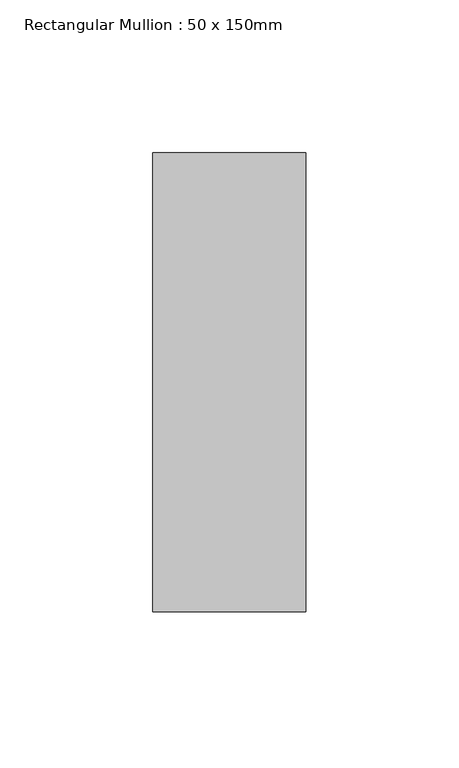
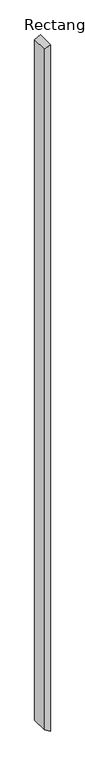
"""IFC4 building model written with IfcOpenShell, lengths in millimetres: member geometry, Rectangular Mullion : 50 x 150mm."""

from ifc_helpers import new_model, si_unit, frame, origin, place, context, project, spatial, polyline, outline, extrude, source, transform, mapped, element, save


def rectangular_mullion_50_x_150mm_85ac93d7(model_context):
    return source(origin(), model_context, "Body", "SweptSolid", [
        extrude(outline(polyline([(0.0, 0.0), (-25.8377402, -50.0), (-6312.9528574, -50.0), (-6342.8393821, 0.0), (0.0, 0.0)])), frame((0.0, -75.0, 0.0), z_axis=(0.0, 1.0, 0.0), x_axis=(0.0, 0.0, 1.0)), (0.0, 0.0, 1.0), 150.0),
    ])


if __name__ == "__main__":
    model = new_model("IFC4")
    model_context = context("Model", 3, world=origin())
    ifc_project = project(units=[si_unit("LENGTHUNIT", "METRE", prefix="MILLI")], contexts=[model_context])
    site = spatial("IfcSite", under=ifc_project)
    building = spatial("IfcBuilding", under=site)
    placement = place(None, origin())
    rectangular_mullion_50_x_150mm_shape = rectangular_mullion_50_x_150mm_85ac93d7(model_context)
    element("IfcMember", 1, ObjectType="Rectangular Mullion : 50 x 150mm", at=placement, inside=building, context=model_context, shape_type="MappedRepresentation", body=[
        mapped(rectangular_mullion_50_x_150mm_shape, transform((0.0, 0.0, 0.0), x_axis=(1.0, 0.0, 0.0), y_axis=(0.0, 1.0, 0.0), z_axis=(0.0, 0.0, 1.0))),
    ])
    save(model, "model.ifc")

# Revit data of these elements
# Type "Rectangular Mullion : 50 x 150mm"
#   built-in parameter 1007304 = 0.492126 (stored number, unit not read)
#   built-in parameter 1007301 = 0.082021 (stored number, unit not read)
#   built-in parameter 1007300 = 0.082021 (stored number, unit not read)
# Element 1 (IfcMember, "Rectangular Mullion : 50 x 150mm")
#   Materials on its faces: "Metal - Aluminium"
# Materials
#   "Metal - Aluminium": class "Metal", colour RGB 247 247 247, transparency 0
